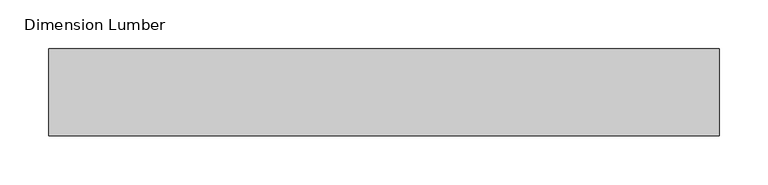
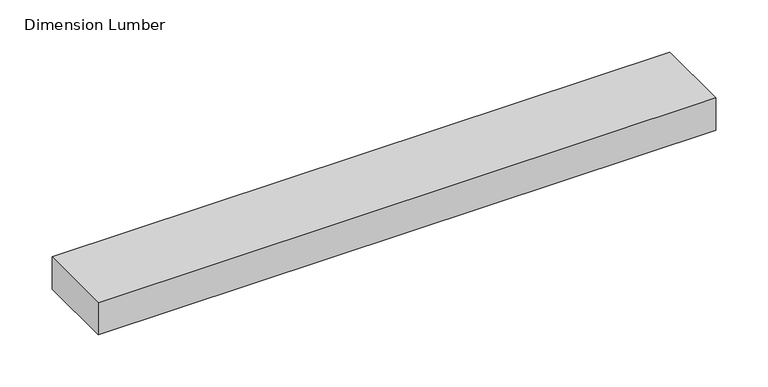
"""IFC4 building model written with IfcOpenShell, lengths in millimetres: beam geometry, Dimension Lumber : Opening Plate 2*4 Exterior."""

from ifc_helpers import new_model, si_unit, frame, origin, place, context, project, spatial, polyline, outline, extrude, source, transform, mapped, element, save


def dimension_lumber_e295fb9e(model_context):
    return source(origin(), model_context, "Body", "SweptSolid", [
        extrude(outline(polyline([(333.375, 44.45), (333.375, -44.45), (-352.4249994, -44.45), (-352.4249994, 44.45), (333.375, 44.45)])), frame((0.0, 0.0, -19.05), z_axis=(0.0, 0.0, 1.0), x_axis=(1.0, 0.0, 0.0)), (0.0, 0.0, 1.0), 38.1),
    ])


if __name__ == "__main__":
    model = new_model("IFC4")
    model_context = context("Model", 3, world=origin())
    ifc_project = project(units=[si_unit("LENGTHUNIT", "METRE", prefix="MILLI")], contexts=[model_context])
    site = spatial("IfcSite", under=ifc_project)
    building = spatial("IfcBuilding", under=site)
    placement = place(None, origin())
    dimension_lumber_shape = dimension_lumber_e295fb9e(model_context)
    element("IfcBeam", 1, ObjectType="Dimension Lumber : Opening Plate 2*4 Exterior", at=placement, inside=building, context=model_context, shape_type="MappedRepresentation", body=[
        mapped(dimension_lumber_shape, transform((0.0, 0.0, 0.0), x_axis=(1.0, 0.0, 0.0), y_axis=(0.0, 1.0, 0.0), z_axis=(0.0, 0.0, 1.0))),
    ])
    save(model, "model.ifc")

# Revit data of these elements
# Type "Dimension Lumber : Opening Plate 2*4 Exterior"
#   Assembly Code = "B10"
#   A = 0.0364583 SF
#   Length [instance default] = 5' - 0"
#   b = 0' - 3 1/2"
#   d = 0' - 1 1/2"
#   Structural Material [instance default] = Softwood, Lumber
# Element 1 (IfcBeam, "Dimension Lumber : Opening Plate 2*4 Exterior")
#   Structural Material = Douglas Fir #2
#   Materials on its faces: "Douglas Fir #2"
# Materials
#   "Softwood, Lumber": class "Wood", colour RGB 223 192 134, transparency 0, Description = "Pinus Echinata", Cost = 0
#   "Douglas Fir #2": class "Wood", colour RGB 223 192 134, transparency 0, Description = "Pinus Echinata", Cost = 0
